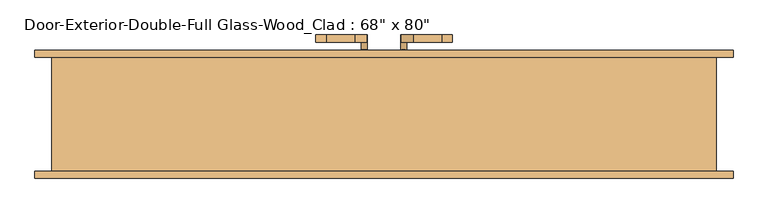
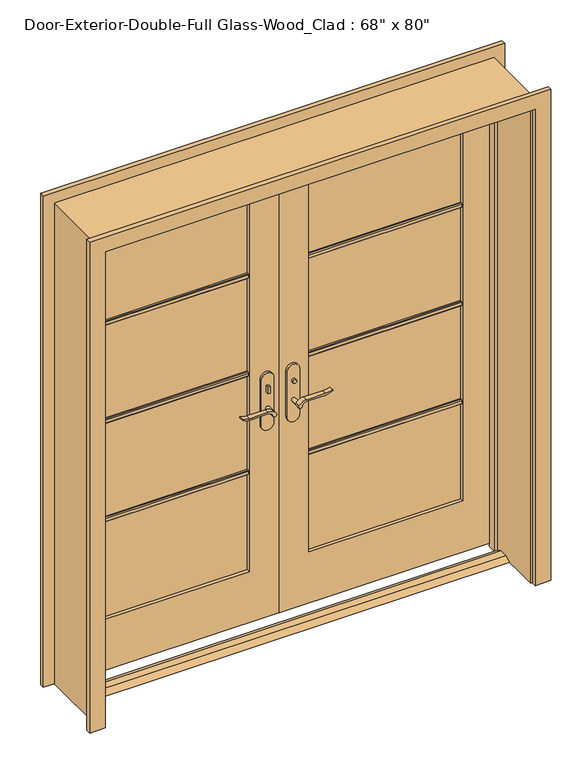
"""IFC4 building model written with IfcOpenShell, lengths in millimetres: door geometry."""

from ifc_helpers import new_model, si_unit, point, frame, frame_2d, origin, place, context, project, spatial, polyline, circle_curve, trimmed, segment, composite_curve, outline, extrude, faceted_brep, source, transform, mapped, element, save


def door_f3362da7(model_context):
    return source(origin(), model_context, "Body", "SolidModel", [
        extrude(outline(polyline([(19.05, 12.7), (53.975, 12.7), (79.375, 0.0), (-6.35, 0.0), (19.05, 12.7)])), frame((-863.6, 0.0, 0.0), z_axis=(1.0, 0.0, 0.0), x_axis=(0.0, 1.0, 0.0)), (0.0, 0.0, 1.0), 1727.2),
        extrude(outline(polyline([(-47.4019111, 94.3), (-57.4019111, 94.3), (-57.4019111, 104.3), (-47.4019111, 104.3), (-47.4019111, 94.3)])), frame((0.0, 0.0, 981.9), z_axis=(0.0, 0.0, 1.0), x_axis=(1.0, 0.0, 0.0)), (0.0, 0.0, 1.0), 30.0),
        extrude(outline(composite_curve([segment(trimmed(circle_curve(frame_2d((996.9, -52.4019111)), 8.0), [point((996.9, -60.4019111))], [point((996.9, -44.4019111))], False, "CARTESIAN"), True, "CONTINUOUS"), segment(trimmed(circle_curve(frame_2d((996.9, -52.4019111)), 8.0), [point((996.9, -44.4019111))], [point((996.9, -60.4019111))], False, "CARTESIAN"), True, "CONTINUOUS")], self_intersect=False)), frame((0.0, 159.225, 0.0), z_axis=(0.0, 1.0, 0.0), x_axis=(0.0, 0.0, 1.0)), (0.0, 0.0, 1.0), 10.0),
        extrude(outline(composite_curve([segment(trimmed(circle_curve(frame_2d((897.1555521, -76.0694241)), 37.2832219), [point((919.0523287, -45.8937749))], [point((934.4, -77.7693445))], False, "CARTESIAN"), True, "CONTINUOUS"), segment(polyline([(934.4, -77.7693445), (934.4, -154.045502)]), True, "CONTINUOUS"), segment(trimmed(circle_curve(frame_2d((1017.6850638, -153.9791202)), 83.2850902), [point((934.4, -154.045502))], [point((939.4, -182.4019111))], True, "CARTESIAN"), True, "CONTINUOUS"), segment(polyline([(939.4, -182.4019111), (936.6135558, -182.4019111)]), True, "CONTINUOUS"), segment(trimmed(circle_curve(frame_2d((986.6709207, -150.4622499)), 59.3791355), [point((936.6135558, -182.4019111))], [point((927.4, -154.045502))], False, "CARTESIAN"), True, "CONTINUOUS"), segment(polyline([(927.4, -154.045502), (927.4, -77.7881013)]), True, "CONTINUOUS"), segment(trimmed(circle_curve(frame_2d((909.2738613, -77.7881013)), 18.1261387), [point((927.4, -77.7881013))], [point((914.4, -60.4019111))], True, "CARTESIAN"), True, "CONTINUOUS"), segment(trimmed(circle_curve(frame_2d((914.4, -52.4019111)), 8.0), [point((914.4, -60.4019111))], [point((919.0523287, -45.8937749))], False, "CARTESIAN"), True, "CONTINUOUS")], self_intersect=False)), frame((0.0, 54.3, 0.0), z_axis=(0.0, 1.0, 0.0), x_axis=(0.0, 0.0, 1.0)), (0.0, 0.0, 1.0), 20.0),
        extrude(outline(composite_curve([segment(trimmed(circle_curve(frame_2d((914.4, -52.4019111)), 8.0), [point((914.3999903, -60.4019111))], [point((919.0523287, -45.8937749))], False, "CARTESIAN"), True, "CONTINUOUS"), segment(trimmed(circle_curve(frame_2d((897.1555521, -76.0694241)), 37.2832219), [point((919.0523287, -45.8937749))], [point((934.4, -77.7693445))], False, "CARTESIAN"), True, "CONTINUOUS"), segment(polyline([(934.4, -77.7693445), (934.4, -154.045502)]), True, "CONTINUOUS"), segment(trimmed(circle_curve(frame_2d((1017.6850638, -153.9791202)), 83.2850902), [point((934.4, -154.045502))], [point((939.4, -182.4019111))], True, "CARTESIAN"), True, "CONTINUOUS"), segment(polyline([(939.4, -182.4019111), (936.6135558, -182.4019111)]), True, "CONTINUOUS"), segment(trimmed(circle_curve(frame_2d((986.6709207, -150.4622499)), 59.3791355), [point((936.6135558, -182.4019111))], [point((927.4, -154.045502))], False, "CARTESIAN"), True, "CONTINUOUS"), segment(polyline([(927.4, -154.045502), (927.4, -77.788099)]), True, "CONTINUOUS"), segment(trimmed(circle_curve(frame_2d((909.2738682, -77.788099)), 18.1261318), [point((927.4, -77.788099))], [point((914.3999903, -60.4019111))], True, "CARTESIAN"), True, "CONTINUOUS")], self_intersect=False)), frame((0.0, 189.225, 0.0), z_axis=(0.0, 1.0, 0.0), x_axis=(0.0, 0.0, 1.0)), (0.0, 0.0, 1.0), 20.0),
        extrude(outline(composite_curve([segment(trimmed(circle_curve(frame_2d((914.4, -52.4019111)), 8.0), [point((914.4, -60.4019111))], [point((914.4, -44.4019111))], False, "CARTESIAN"), True, "CONTINUOUS"), segment(trimmed(circle_curve(frame_2d((914.4, -52.4019111)), 8.0), [point((914.4, -44.4019111))], [point((914.4, -60.4019111))], False, "CARTESIAN"), True, "CONTINUOUS")], self_intersect=False)), frame((0.0, 74.3, 0.0), z_axis=(0.0, 1.0, 0.0), x_axis=(0.0, 0.0, 1.0)), (0.0, 0.0, 1.0), 30.0),
        extrude(outline(composite_curve([segment(trimmed(circle_curve(frame_2d((914.4, -52.4019111)), 8.0), [point((914.4, -60.4019111))], [point((914.4, -44.4019111))], False, "CARTESIAN"), True, "CONTINUOUS"), segment(trimmed(circle_curve(frame_2d((914.4, -52.4019111)), 8.0), [point((914.4, -44.4019111))], [point((914.4, -60.4019111))], False, "CARTESIAN"), True, "CONTINUOUS")], self_intersect=False)), frame((0.0, 159.225, 0.0), z_axis=(0.0, 1.0, 0.0), x_axis=(0.0, 0.0, 1.0)), (0.0, 0.0, 1.0), 30.0),
        extrude(outline(composite_curve([segment(polyline([(844.4, -27.4019111), (1039.4, -27.4019111)]), True, "CONTINUOUS"), segment(trimmed(circle_curve(frame_2d((1039.4, -52.4019111)), 25.0), [point((1039.4, -27.4019111))], [point((1039.4, -77.4019111))], False, "CARTESIAN"), True, "CONTINUOUS"), segment(polyline([(1039.4, -77.4019111), (844.4, -77.4019111)]), True, "CONTINUOUS"), segment(trimmed(circle_curve(frame_2d((844.4, -52.4019111)), 25.0), [point((844.4, -77.4019111))], [point((844.4, -27.4019111))], False, "CARTESIAN"), True, "CONTINUOUS")], self_intersect=False)), frame((0.0, 104.3, 0.0), z_axis=(0.0, 1.0, 0.0), x_axis=(0.0, 0.0, 1.0)), (0.0, 0.0, 1.0), 10.0),
        extrude(outline(composite_curve([segment(polyline([(844.4, -27.4019111), (1039.4, -27.4019111)]), True, "CONTINUOUS"), segment(trimmed(circle_curve(frame_2d((1039.4, -52.4019111)), 25.0), [point((1039.4, -27.4019111))], [point((1039.4, -77.4019111))], False, "CARTESIAN"), True, "CONTINUOUS"), segment(polyline([(1039.4, -77.4019111), (844.4, -77.4019111)]), True, "CONTINUOUS"), segment(trimmed(circle_curve(frame_2d((844.4, -52.4019111)), 25.0), [point((844.4, -77.4019111))], [point((844.4, -27.4019111))], False, "CARTESIAN"), True, "CONTINUOUS")], self_intersect=False)), frame((0.0, 149.225, 0.0), z_axis=(0.0, 1.0, 0.0), x_axis=(0.0, 0.0, 1.0)), (0.0, 0.0, 1.0), 10.0),
        extrude(outline(polyline([(47.3875, 169.225), (57.3875, 169.225), (57.3875, 159.225), (47.3875, 159.225), (47.3875, 169.225)])), frame((0.0, 0.0, 981.9), z_axis=(0.0, 0.0, 1.0), x_axis=(1.0, 0.0, 0.0)), (0.0, 0.0, 1.0), 30.0),
        extrude(outline(composite_curve([segment(trimmed(circle_curve(frame_2d((996.9, 52.3875)), 8.0), [point((996.9, 60.3875))], [point((996.9, 44.3875))], False, "CARTESIAN"), True, "CONTINUOUS"), segment(trimmed(circle_curve(frame_2d((996.9, 52.3875)), 8.0), [point((996.9, 44.3875))], [point((996.9, 60.3875))], False, "CARTESIAN"), True, "CONTINUOUS")], self_intersect=False)), frame((0.0, 94.3, 0.0), z_axis=(0.0, 1.0, 0.0), x_axis=(0.0, 0.0, 1.0)), (0.0, 0.0, 1.0), 10.0),
        extrude(outline(composite_curve([segment(trimmed(circle_curve(frame_2d((914.4, 52.3875)), 8.0), [point((919.0523287, 45.8793637))], [point((914.4, 60.3875))], False, "CARTESIAN"), True, "CONTINUOUS"), segment(trimmed(circle_curve(frame_2d((909.2738613, 77.7736901)), 18.1261387), [point((914.4, 60.3875))], [point((927.4, 77.7736901))], True, "CARTESIAN"), True, "CONTINUOUS"), segment(polyline([(927.4, 77.7736901), (927.4, 154.0310909)]), True, "CONTINUOUS"), segment(trimmed(circle_curve(frame_2d((986.6709207, 150.4478388)), 59.3791355), [point((927.4, 154.0310909))], [point((936.6135558, 182.3875))], False, "CARTESIAN"), True, "CONTINUOUS"), segment(polyline([(936.6135558, 182.3875), (939.4, 182.3875)]), True, "CONTINUOUS"), segment(trimmed(circle_curve(frame_2d((1017.6850638, 153.9647091)), 83.2850902), [point((939.4, 182.3875))], [point((934.4, 154.0310909))], True, "CARTESIAN"), True, "CONTINUOUS"), segment(polyline([(934.4, 154.0310909), (934.4, 77.7549333)]), True, "CONTINUOUS"), segment(trimmed(circle_curve(frame_2d((897.1555521, 76.0550129)), 37.2832219), [point((934.4, 77.7549333))], [point((919.0523287, 45.8793637))], False, "CARTESIAN"), True, "CONTINUOUS")], self_intersect=False)), frame((0.0, 189.225, 0.0), z_axis=(0.0, 1.0, 0.0), x_axis=(0.0, 0.0, 1.0)), (0.0, 0.0, 1.0), 20.0),
        extrude(outline(composite_curve([segment(trimmed(circle_curve(frame_2d((909.2738682, 77.7736878)), 18.1261318), [point((914.3999903, 60.3875))], [point((927.4, 77.7736878))], True, "CARTESIAN"), True, "CONTINUOUS"), segment(polyline([(927.4, 77.7736878), (927.4, 154.0310909)]), True, "CONTINUOUS"), segment(trimmed(circle_curve(frame_2d((986.6709207, 150.4478388)), 59.3791355), [point((927.4, 154.0310909))], [point((936.6135558, 182.3875))], False, "CARTESIAN"), True, "CONTINUOUS"), segment(polyline([(936.6135558, 182.3875), (939.4, 182.3875)]), True, "CONTINUOUS"), segment(trimmed(circle_curve(frame_2d((1017.6850638, 153.9647091)), 83.2850902), [point((939.4, 182.3875))], [point((934.4, 154.0310909))], True, "CARTESIAN"), True, "CONTINUOUS"), segment(polyline([(934.4, 154.0310909), (934.4, 77.7549333)]), True, "CONTINUOUS"), segment(trimmed(circle_curve(frame_2d((897.1555521, 76.0550129)), 37.2832219), [point((934.4, 77.7549333))], [point((919.0523287, 45.8793637))], False, "CARTESIAN"), True, "CONTINUOUS"), segment(trimmed(circle_curve(frame_2d((914.4, 52.3875)), 8.0), [point((919.0523287, 45.8793637))], [point((914.3999903, 60.3875))], False, "CARTESIAN"), True, "CONTINUOUS")], self_intersect=False)), frame((0.0, 54.3, 0.0), z_axis=(0.0, 1.0, 0.0), x_axis=(0.0, 0.0, 1.0)), (0.0, 0.0, 1.0), 20.0),
        extrude(outline(composite_curve([segment(trimmed(circle_curve(frame_2d((914.4, 52.3875)), 8.0), [point((914.4, 60.3875))], [point((914.4, 44.3875))], False, "CARTESIAN"), True, "CONTINUOUS"), segment(trimmed(circle_curve(frame_2d((914.4, 52.3875)), 8.0), [point((914.4, 44.3875))], [point((914.4, 60.3875))], False, "CARTESIAN"), True, "CONTINUOUS")], self_intersect=False)), frame((0.0, 159.225, 0.0), z_axis=(0.0, 1.0, 0.0), x_axis=(0.0, 0.0, 1.0)), (0.0, 0.0, 1.0), 30.0),
        extrude(outline(composite_curve([segment(trimmed(circle_curve(frame_2d((914.4, 52.3875)), 8.0), [point((914.4, 60.3875))], [point((914.4, 44.3875))], False, "CARTESIAN"), True, "CONTINUOUS"), segment(trimmed(circle_curve(frame_2d((914.4, 52.3875)), 8.0), [point((914.4, 44.3875))], [point((914.4, 60.3875))], False, "CARTESIAN"), True, "CONTINUOUS")], self_intersect=False)), frame((0.0, 74.3, 0.0), z_axis=(0.0, 1.0, 0.0), x_axis=(0.0, 0.0, 1.0)), (0.0, 0.0, 1.0), 30.0),
        extrude(outline(composite_curve([segment(trimmed(circle_curve(frame_2d((844.4, 52.3875)), 25.0), [point((844.4, 27.3875))], [point((844.4, 77.3875))], False, "CARTESIAN"), True, "CONTINUOUS"), segment(polyline([(844.4, 77.3875), (1039.4, 77.3875)]), True, "CONTINUOUS"), segment(trimmed(circle_curve(frame_2d((1039.4, 52.3875)), 25.0), [point((1039.4, 77.3875))], [point((1039.4, 27.3875))], False, "CARTESIAN"), True, "CONTINUOUS"), segment(polyline([(1039.4, 27.3875), (844.4, 27.3875)]), True, "CONTINUOUS")], self_intersect=False)), frame((0.0, 149.225, 0.0), z_axis=(0.0, 1.0, 0.0), x_axis=(0.0, 0.0, 1.0)), (0.0, 0.0, 1.0), 10.0),
        extrude(outline(composite_curve([segment(trimmed(circle_curve(frame_2d((844.4, 52.3875)), 25.0), [point((844.4, 27.3875))], [point((844.4, 77.3875))], False, "CARTESIAN"), True, "CONTINUOUS"), segment(polyline([(844.4, 77.3875), (1039.4, 77.3875)]), True, "CONTINUOUS"), segment(trimmed(circle_curve(frame_2d((1039.4, 52.3875)), 25.0), [point((1039.4, 77.3875))], [point((1039.4, 27.3875))], False, "CARTESIAN"), True, "CONTINUOUS"), segment(polyline([(1039.4, 27.3875), (844.4, 27.3875)]), True, "CONTINUOUS")], self_intersect=False)), frame((0.0, 104.3, 0.0), z_axis=(0.0, 1.0, 0.0), x_axis=(0.0, 0.0, 1.0)), (0.0, 0.0, 1.0), 10.0),
        extrude(outline(polyline([(128.27, 1502.171875), (128.27, 1483.121875), (121.92, 1483.121875), (118.745, 1486.296875), (118.745, 1498.996875), (121.92, 1502.171875), (128.27, 1502.171875)])), frame((120.65, 0.0, 0.0), z_axis=(1.0, 0.0, 0.0), x_axis=(0.0, 1.0, 0.0)), (0.0, 0.0, 1.0), 622.3),
        extrude(outline(polyline([(128.27, 1081.88125), (128.27, 1062.83125), (121.92, 1062.83125), (118.745, 1066.00625), (118.745, 1078.70625), (121.92, 1081.88125), (128.27, 1081.88125)])), frame((120.65, 0.0, 0.0), z_axis=(1.0, 0.0, 0.0), x_axis=(0.0, 1.0, 0.0)), (0.0, 0.0, 1.0), 622.3),
        extrude(outline(polyline([(128.27, 661.590625), (128.27, 642.540625), (121.92, 642.540625), (118.745, 645.715625), (118.745, 658.415625), (121.92, 661.590625), (128.27, 661.590625)])), frame((120.65, 0.0, 0.0), z_axis=(1.0, 0.0, 0.0), x_axis=(0.0, 1.0, 0.0)), (0.0, 0.0, 1.0), 622.3),
        extrude(outline(polyline([(135.255, 1502.171875), (141.605, 1502.171875), (144.78, 1498.996875), (144.78, 1486.296875), (141.605, 1483.121875), (135.255, 1483.121875), (135.255, 1502.171875)])), frame((-742.95, 0.0, 0.0), z_axis=(1.0, 0.0, 0.0), x_axis=(0.0, 1.0, 0.0)), (0.0, 0.0, 1.0), 622.3),
        extrude(outline(polyline([(135.255, 1081.88125), (141.605, 1081.88125), (144.78, 1078.70625), (144.78, 1066.00625), (141.605, 1062.83125), (135.255, 1062.83125), (135.255, 1081.88125)])), frame((-742.95, 0.0, 0.0), z_axis=(1.0, 0.0, 0.0), x_axis=(0.0, 1.0, 0.0)), (0.0, 0.0, 1.0), 622.3),
        extrude(outline(polyline([(135.255, 661.590625), (141.605, 661.590625), (144.78, 658.415625), (144.78, 645.715625), (141.605, 642.540625), (135.255, 642.540625), (135.255, 661.590625)])), frame((-742.95, 0.0, 0.0), z_axis=(1.0, 0.0, 0.0), x_axis=(0.0, 1.0, 0.0)), (0.0, 0.0, 1.0), 622.3),
        extrude(outline(polyline([(135.255, 1502.171875), (141.605, 1502.171875), (144.78, 1498.996875), (144.78, 1486.296875), (141.605, 1483.121875), (135.255, 1483.121875), (135.255, 1502.171875)])), frame((120.65, 0.0, 0.0), z_axis=(1.0, 0.0, 0.0), x_axis=(0.0, 1.0, 0.0)), (0.0, 0.0, 1.0), 622.3),
        extrude(outline(polyline([(135.255, 1081.88125), (141.605, 1081.88125), (144.78, 1078.70625), (144.78, 1066.00625), (141.605, 1062.83125), (135.255, 1062.83125), (135.255, 1081.88125)])), frame((120.65, 0.0, 0.0), z_axis=(1.0, 0.0, 0.0), x_axis=(0.0, 1.0, 0.0)), (0.0, 0.0, 1.0), 622.3),
        extrude(outline(polyline([(135.255, 661.590625), (141.605, 661.590625), (144.78, 658.415625), (144.78, 645.715625), (141.605, 642.540625), (135.255, 642.540625), (135.255, 661.590625)])), frame((120.65, 0.0, 0.0), z_axis=(1.0, 0.0, 0.0), x_axis=(0.0, 1.0, 0.0)), (0.0, 0.0, 1.0), 622.3),
        extrude(outline(polyline([(128.27, 1502.171875), (128.27, 1483.121875), (121.92, 1483.121875), (118.745, 1486.296875), (118.745, 1498.996875), (121.92, 1502.171875), (128.27, 1502.171875)])), frame((-742.95, 0.0, 0.0), z_axis=(1.0, 0.0, 0.0), x_axis=(0.0, 1.0, 0.0)), (0.0, 0.0, 1.0), 622.3),
        extrude(outline(polyline([(128.27, 1081.88125), (128.27, 1062.83125), (121.92, 1062.83125), (118.745, 1066.00625), (118.745, 1078.70625), (121.92, 1081.88125), (128.27, 1081.88125)])), frame((-742.95, 0.0, 0.0), z_axis=(1.0, 0.0, 0.0), x_axis=(0.0, 1.0, 0.0)), (0.0, 0.0, 1.0), 622.3),
        extrude(outline(polyline([(128.27, 661.590625), (128.27, 642.540625), (121.92, 642.540625), (118.745, 645.715625), (118.745, 658.415625), (121.92, 661.590625), (128.27, 661.590625)])), frame((-742.95, 0.0, 0.0), z_axis=(1.0, 0.0, 0.0), x_axis=(0.0, 1.0, 0.0)), (0.0, 0.0, 1.0), 622.3),
        extrude(outline(polyline([(0.0, 869.95), (0.0, 933.45), (2101.85, 933.45), (2101.85, -933.45), (0.0, -933.45), (0.0, -869.95), (2038.35, -869.95), (2038.35, 869.95), (0.0, 869.95)])), frame((0.0, 149.225, 0.0), z_axis=(0.0, 1.0, 0.0), x_axis=(0.0, 0.0, 1.0)), (0.0, 0.0, 1.0), 19.05),
        extrude(outline(polyline([(0.0, 869.95), (0.0, 933.45), (2101.85, 933.45), (2101.85, -933.45), (0.0, -933.45), (0.0, -869.95), (2038.35, -869.95), (2038.35, 869.95), (0.0, 869.95)])), frame((0.0, -174.625, 0.0), z_axis=(0.0, 1.0, 0.0), x_axis=(0.0, 0.0, 1.0)), (0.0, 0.0, 1.0), 19.05),
        extrude(outline(polyline([(12.7, 863.6), (2032.0, 863.6), (2032.0, 1.5875), (12.7, 1.5875), (12.7, 863.6)]), holes=[polyline([(1912.9375, 120.65), (1912.9375, 742.95), (231.775, 742.95), (231.775, 120.65), (1912.9375, 120.65)])]), frame((0.0, 114.3, 0.0), z_axis=(0.0, 1.0, 0.0), x_axis=(0.0, 0.0, 1.0)), (0.0, 0.0, 1.0), 34.925),
        extrude(outline(polyline([(2032.0, -863.6), (12.7, -863.6), (12.7, -1.6019111), (2032.0, -1.6019111), (2032.0, -863.6)]), holes=[polyline([(231.775, -742.95), (1912.9375, -742.95), (1912.9375, -120.65), (231.775, -120.65), (231.775, -742.95)])]), frame((0.0, 114.3, 0.0), z_axis=(0.0, 1.0, 0.0), x_axis=(0.0, 0.0, 1.0)), (0.0, 0.0, 1.0), 34.925),
        faceted_brep([(889.0, 149.225, 0.0), (889.0, -155.575, 0.0), (863.6, -155.575, 0.0), (863.6, 79.375, 0.0), (850.9, 79.375, 0.0), (850.9, 114.3, 0.0), (863.6, 114.3, 0.0), (863.6, 149.225, 0.0), (889.0, 149.225, 2057.4), (889.0, -155.575, 2057.4), (-889.0, -155.575, 2057.4), (-889.0, -155.575, 0.0), (-863.6, -155.575, 0.0), (-863.6, -155.575, 2032.0), (863.6, -155.575, 2032.0), (863.6, 79.375, 2032.0), (-863.6, 79.375, 2032.0), (-863.6, 79.375, 0.0), (-850.9, 79.375, 0.0), (-850.9, 79.375, 2019.3), (850.9, 79.375, 2019.3), (850.9, 114.3, 2019.3), (1.5875, 114.3, 2019.3), (-1.6019111, 114.3, 2019.3), (-850.9, 114.3, 2019.3), (-850.9, 114.3, 0.0), (-863.6, 114.3, 0.0), (-863.6, 114.3, 2032.0), (-1.6019111, 114.3, 2032.0), (1.5875, 114.3, 2032.0), (863.6, 114.3, 2032.0), (863.6, 149.225, 2032.0), (1.5875, 149.225, 2032.0), (-1.6019111, 149.225, 2032.0), (-863.6, 149.225, 2032.0), (-863.6, 149.225, 0.0), (-889.0, 149.225, 0.0), (-889.0, 149.225, 2057.4)], [[[0, 1, 2, 3, 4, 5, 6, 7]], [[1, 0, 8, 9]], [[2, 1, 9, 10, 11, 12, 13, 14]], [[3, 2, 14, 15]], [[4, 3, 15, 16, 17, 18, 19, 20]], [[5, 4, 20, 21]], [[6, 5, 21, 22, 23, 24, 25, 26, 27, 28, 29, 30]], [[7, 6, 30, 31]], [[0, 7, 31, 32, 33, 34, 35, 36, 37, 8]], [[9, 8, 37, 10]], [[14, 13, 16, 15]], [[20, 19, 24, 23, 22, 21]], [[31, 30, 29, 28, 27, 34, 33, 32]], [[12, 11, 36, 35, 26, 25, 18, 17]], [[11, 10, 37, 36]], [[13, 12, 17, 16]], [[19, 18, 25, 24]], [[27, 26, 35, 34]]]),
        extrude(outline(polyline([(742.95, 128.27), (120.65, 128.27), (120.65, 135.255), (742.95, 135.255), (742.95, 128.27)])), frame((0.0, 0.0, 231.775), z_axis=(0.0, 0.0, 1.0), x_axis=(1.0, 0.0, 0.0)), (0.0, 0.0, 1.0), 1681.1625),
        extrude(outline(polyline([(-120.65, 128.27), (-742.95, 128.27), (-742.95, 135.255), (-120.65, 135.255), (-120.65, 128.27)])), frame((0.0, 0.0, 231.775), z_axis=(0.0, 0.0, 1.0), x_axis=(1.0, 0.0, 0.0)), (0.0, 0.0, 1.0), 1681.1625),
    ])


if __name__ == "__main__":
    model = new_model("IFC4")
    model_context = context("Model", 3, world=origin())
    ifc_project = project(units=[si_unit("LENGTHUNIT", "METRE", prefix="MILLI")], contexts=[model_context])
    site = spatial("IfcSite", under=ifc_project)
    building = spatial("IfcBuilding", under=site)
    placement = place(None, origin())
    door_shape = door_f3362da7(model_context)
    element("IfcDoor", 1, ObjectType="Door-Exterior-Double-Full Glass-Wood_Clad : 68\" x 80\"", at=placement, inside=building, context=model_context, shape_type="MappedRepresentation", body=[
        mapped(door_shape, transform((0.0, 0.0, 0.0), x_axis=(1.0, 0.0, 0.0), y_axis=(0.0, 1.0, 0.0), z_axis=(0.0, 0.0, 1.0))),
    ])
    save(model, "model.ifc")

# Revit data of these elements
# Type "Door-Exterior-Double-Full Glass-Wood_Clad : 68\" x 80\""
#   Type Mark = "21"
#   Assembly Code = "B2030100"
#   Analytic Construction = "French door, wood frame with double glass"
#   Top Rail = 0' - 4 11/16"
#   Threshold Offset [instance default] = 0' - 0 1/2"
#   Thickness = 0' - 1 3/8"
#   Thermal Resistance (R) = 1.9158 (h·ft²·°F)/BTU
#   Swing Angle [instance default] = 90.0000°
#   Stiles = 0' - 4 3/4"
#   Rough Width = 5' - 10"
#   Rough Height = 6' - 9"
#   Panel Width = 2' - 10"
#   Door Offset [instance default] = 0' - 0"
#   Height = 6' - 8"
#   Width = 5' - 8"
#   Heat Transfer Coefficient (U) = 0.5220 BTU/(h·ft²·°F)
#   Bottom Rail = 0' - 9 1/8"
#   Exterior Trim [instance default] = yes
#   Threshold [instance default] = yes
#   Show Grill [instance default] = yes
#   Function = 1
#   Trim Material = Clad - White
#   Threshold Material = Maple - Semigloss(Rotated)
#   Panel Material = Clad - White
#   Glazing = Glass, Clear Glazing
#   Frame Material = Clad - White
#   Door Handle Material = Aluminum
#   Visual Light Transmittance = 0
#   Solar Heat Gain Coefficient = 0
#   Wall Closure = (empty or 0)
#   Construction Type = (empty or 0)
# Element 1 (IfcDoor, "Door-Exterior-Double-Full Glass-Wood_Clad : 68\" x 80\"")
#   Materials on its faces: "Clad - White", "Aluminum", "Glass, Clear Glazing", "Maple - Semigloss(Rotated)"
# Materials
#   "Clad - White": class "Wood", colour RGB 245 245 243, transparency 0, Cost = 0
#   "Maple - Semigloss(Rotated)": class "Wood", colour RGB 196 161 118, transparency 0, Description = "Acer Saccharum", Cost = 0
#   "Glass, Clear Glazing": class "Glass", colour RGB 245 245 243, transparency 1, Description = "Clear glazing", Cost = 0
#   "Aluminum": class "Metal", colour RGB 244 245 246, transparency 0, Description = "Aluminum 6061", Cost = 0
